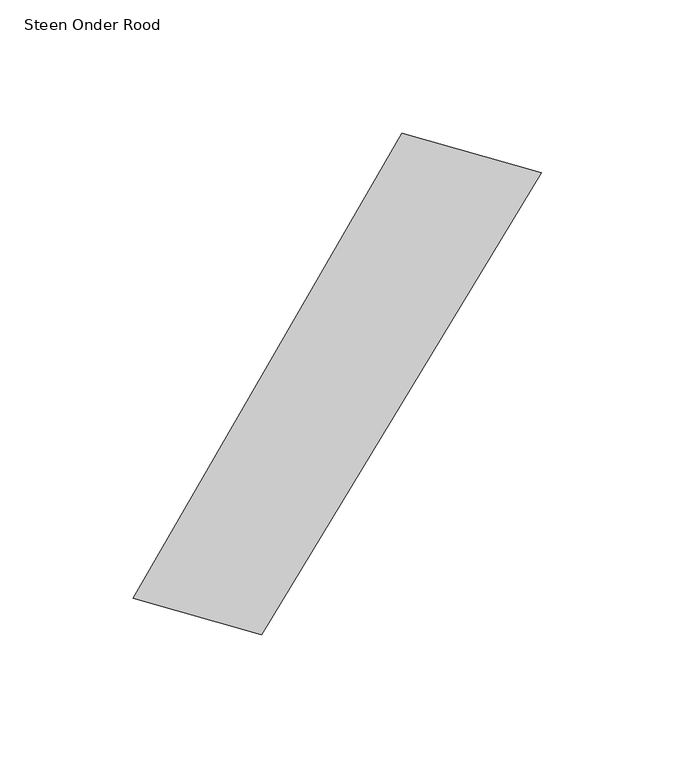
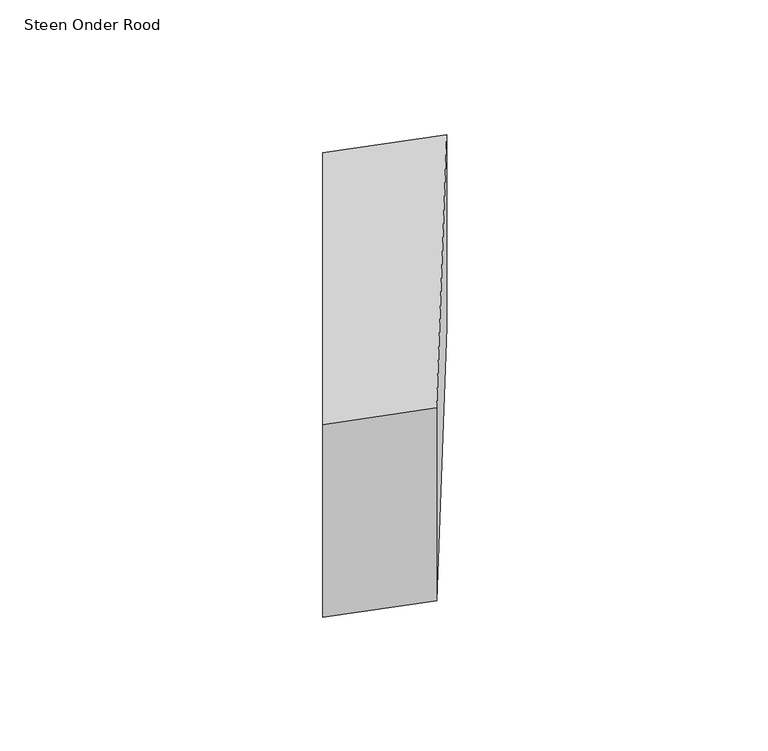
"""IFC4 building model written with IfcOpenShell, lengths in millimetres: proxy geometry, 00_GMA_steen_versie_4 : Steen Onder Rood."""

import ifcopenshell
import ifcopenshell.guid

model = None  # the IFC model being written
_history = None  # IfcOwnerHistory: only IFC2X3 demands one
_inside = {}  # id of a spatial element -> (the spatial element, [elements in it])
_under = {}  # id of a project, library or spatial element -> (it, [spatial elements below it])
_declared = {}  # id of a project -> (the project, [libraries it declares])
_typed = {}  # id of a type object -> (the type object, [elements of that type])
_made_of = {}  # id of a material, layer set ... -> (it, [elements and type objects made of it])


def new_model(schema):
    """Start an empty IFC model of exactly this schema.

    Asked for "IFC4X3", IfcOpenShell would pick the latest addendum, in which some entities
    have other attributes; the version numbers below select the first issue.
    IFC2X3 requires an IfcOwnerHistory on every rooted entity: one is made here for all.
    """
    global model, _history
    if schema == "IFC4X3":
        model = ifcopenshell.file(schema_version=(4, 3, 0, 0))
    else:
        model = ifcopenshell.file(schema=schema)
    _inside.clear()
    _under.clear()
    _declared.clear()
    _typed.clear()
    _made_of.clear()
    _history = None
    if model.schema == "IFC2X3":
        org = make("IfcOrganization", Name="unknown")
        user = make(
            "IfcPersonAndOrganization",
            ThePerson=make("IfcPerson", FamilyName="unknown"),
            TheOrganization=org,
        )
        app = make(
            "IfcApplication",
            ApplicationDeveloper=org,
            Version="unknown",
            ApplicationFullName="unknown",
            ApplicationIdentifier="unknown",
        )
        _history = make(
            "IfcOwnerHistory",
            OwningUser=user,
            OwningApplication=app,
            ChangeAction="ADDED",
            CreationDate=0,
        )
    return model


def make(cls, **values):
    """One entity of the class cls with the attributes given. An attribute that is None is left unset."""
    return model.create_entity(
        cls, **{name: value for name, value in values.items() if value is not None}
    )


def rooted(cls, **values):
    """An entity with a GlobalId (a new one), such as an element, a storey or a relation."""
    return make(cls, GlobalId=ifcopenshell.guid.new(), OwnerHistory=_history, **values)


def si_unit(unit_type, name, prefix=None):
    """IfcSIUnit, for example si_unit("LENGTHUNIT", "METRE", prefix="MILLI")."""
    return make("IfcSIUnit", UnitType=unit_type, Prefix=prefix, Name=name)


def assignment(units):
    """IfcUnitAssignment: the units of a project."""
    return None if units is None else make("IfcUnitAssignment", Units=units)


def point(xyz):
    """IfcCartesianPoint."""
    return None if xyz is None else make("IfcCartesianPoint", Coordinates=xyz)


def direction(xyz):
    """IfcDirection."""
    return None if xyz is None else make("IfcDirection", DirectionRatios=xyz)


def frame(location, z_axis=None, x_axis=None):
    """IfcAxis2Placement3D, a coordinate frame: its origin and axes. An axis left out is left unset."""
    return make(
        "IfcAxis2Placement3D",
        Location=point(location),
        Axis=direction(z_axis),
        RefDirection=direction(x_axis),
    )


def origin():
    """The frame at (0, 0, 0) with its axes left unset."""
    return frame((0.0, 0.0, 0.0))


def origin_with_axes():
    """The frame at (0, 0, 0) with the z axis (0, 0, 1) and the x axis (1, 0, 0) written out."""
    return frame((0.0, 0.0, 0.0), z_axis=(0.0, 0.0, 1.0), x_axis=(1.0, 0.0, 0.0))


def place(relative_to, where):
    """IfcLocalPlacement: puts the frame where relative to a parent placement (None: the world)."""
    return make(
        "IfcLocalPlacement", PlacementRelTo=relative_to, RelativePlacement=where
    )


def context(
    kind, dimensions, precision=None, world=None, true_north=None, identifier=None
):
    """IfcGeometricRepresentationContext, for example the 3D "Model" context."""
    return make(
        "IfcGeometricRepresentationContext",
        ContextIdentifier=identifier,
        ContextType=kind,
        CoordinateSpaceDimension=dimensions,
        Precision=precision,
        WorldCoordinateSystem=world,
        TrueNorth=true_north,
    )


def project(units=None, contexts=None):
    """IfcProject with its units and contexts."""
    return rooted(
        "IfcProject",
        Name="project",
        RepresentationContexts=contexts,
        UnitsInContext=assignment(units),
    )


def spatial(cls, under=None, at=None, **own):
    """A site, building, storey or space (cls), placed at a placement, below another one or the project."""
    s = rooted(cls, ObjectPlacement=at, **own)
    if under is not None:
        _under.setdefault(under.id(), (under, []))[1].append(s)
    return s


def polyline(points):
    """IfcPolyline through the points."""
    return make("IfcPolyline", Points=[point(p) for p in points])


def outline(outer, holes=None, kind="AREA"):
    """IfcArbitraryClosedProfileDef: a profile drawn as a closed curve; with holes, ...WithVoids."""
    if holes is None:
        return make("IfcArbitraryClosedProfileDef", ProfileType=kind, OuterCurve=outer)
    return make(
        "IfcArbitraryProfileDefWithVoids",
        ProfileType=kind,
        OuterCurve=outer,
        InnerCurves=holes,
    )


def extrude(swept, where, along, depth):
    """IfcExtrudedAreaSolid: the profile swept, set in the frame where, extruded along a direction by depth."""
    return make(
        "IfcExtrudedAreaSolid",
        SweptArea=swept,
        Position=where,
        ExtrudedDirection=direction(along),
        Depth=depth,
    )


def shape(context_of_items, identifier, shape_type, items):
    """IfcShapeRepresentation: the items that make up one representation, for example the "Body"."""
    return make(
        "IfcShapeRepresentation",
        ContextOfItems=context_of_items,
        RepresentationIdentifier=identifier,
        RepresentationType=shape_type,
        Items=items,
    )


def source(mapping_origin, context_of_items, identifier, shape_type, items):
    """IfcRepresentationMap: a shape defined once, which mapped items show again and again."""
    return make(
        "IfcRepresentationMap",
        MappingOrigin=mapping_origin,
        MappedRepresentation=shape(context_of_items, identifier, shape_type, items),
    )


def transform(
    local_origin,
    x_axis=None,
    y_axis=None,
    z_axis=None,
    scale=None,
    scale2=None,
    scale3=None,
    uniform=True,
):
    """IfcCartesianTransformationOperator3D, or its non-uniform kind. x_axis, y_axis, z_axis: its Axis1, 2, 3."""
    if uniform:
        return make(
            "IfcCartesianTransformationOperator3D",
            Axis1=direction(x_axis),
            Axis2=direction(y_axis),
            LocalOrigin=point(local_origin),
            Scale=scale,
            Axis3=direction(z_axis),
        )
    return make(
        "IfcCartesianTransformationOperator3DnonUniform",
        Axis1=direction(x_axis),
        Axis2=direction(y_axis),
        LocalOrigin=point(local_origin),
        Scale=scale,
        Axis3=direction(z_axis),
        Scale2=scale2,
        Scale3=scale3,
    )


def mapped(mapping_source, mapping_target):
    """IfcMappedItem: shows the shape of a source again, moved by a transform."""
    return make(
        "IfcMappedItem", MappingSource=mapping_source, MappingTarget=mapping_target
    )


def made_of(thing, what):
    """Note that an element or type object is made of a material, layer set ...; save() writes the relation."""
    if what is not None:
        _made_of.setdefault(what.id(), (what, []))[1].append(thing)
    return thing


def element(
    cls,
    number,
    at=None,
    inside=None,
    cuts=None,
    type_object=None,
    material=None,
    context=None,
    identifier="Body",
    shape_type=None,
    held_by="IfcProductDefinitionShape",
    body=None,
    shapes=None,
    **own,
):
    """One element of the class cls, such as IfcWall. Its Tag is "e" and its number.

    at: its placement. inside: the storey or other place that contains it. cuts: it is an
    opening in that element (IfcRelVoidsElement). A single representation is given by context,
    identifier, shape_type and body (its items); several are given by shapes. held_by: the class
    of the entity that holds the representations. save() writes the other relations.
    """
    e = rooted(cls, Tag="e%d" % number, ObjectPlacement=at, **own)
    if body is not None:
        shapes = [shape(context, identifier, shape_type, body)]
    if shapes is not None:
        e.Representation = make(held_by, Representations=shapes)
    if inside is not None:
        _inside.setdefault(inside.id(), (inside, []))[1].append(e)
    if cuts is not None:
        rooted(
            "IfcRelVoidsElement", RelatingBuildingElement=cuts, RelatedOpeningElement=e
        )
    if type_object is not None:
        _typed.setdefault(type_object.id(), (type_object, []))[1].append(e)
    return made_of(e, material)


def aggregate(whole, parts):
    """IfcRelAggregates: a whole, such as a stair, and the parts it consists of."""
    return rooted("IfcRelAggregates", RelatingObject=whole, RelatedObjects=parts)


def save(model, path):
    """Write the relations noted so far, then the file.

    IfcRelAggregates (storeys below a building ...), IfcRelContainedInSpatialStructure (elements
    in a storey), IfcRelDefinesByType, IfcRelAssociatesMaterial and IfcRelDeclares: one each for
    every whole, place, type object, material and project.
    """
    for whole, parts in _under.values():
        aggregate(whole, parts)
    for where, things in _inside.values():
        rooted(
            "IfcRelContainedInSpatialStructure",
            RelatedElements=things,
            RelatingStructure=where,
        )
    for kind, things in _typed.values():
        rooted("IfcRelDefinesByType", RelatedObjects=things, RelatingType=kind)
    for what, things in _made_of.values():
        rooted("IfcRelAssociatesMaterial", RelatedObjects=things, RelatingMaterial=what)
    for by, libraries in _declared.values():
        rooted("IfcRelDeclares", RelatingContext=by, RelatedDefinitions=libraries)
    model.write(path)


def steen_onder_rood_00cee3c2(model_context):
    return source(origin(), model_context, "Body", "SweptSolid", [
        extrude(outline(polyline([(151.9565091, 154.4198212), (46.9301943, -18.7978323), (-1.2031551, -5.2634066), (99.6350154, 169.1084483), (151.9565091, 154.4198212)])), origin_with_axes(), (0.0, 0.0, 1.0), 100.0),
    ])


if __name__ == "__main__":
    model = new_model("IFC4")
    model_context = context("Model", 3, world=origin())
    ifc_project = project(units=[si_unit("LENGTHUNIT", "METRE", prefix="MILLI")], contexts=[model_context])
    site = spatial("IfcSite", under=ifc_project)
    building = spatial("IfcBuilding", under=site)
    placement = place(None, origin())
    steen_onder_rood_shape = steen_onder_rood_00cee3c2(model_context)
    element("IfcBuildingElementProxy", 1, Name="00_GMA_steen_versie_4 : Steen Onder Rood", ObjectType="00_GMA_steen_versie_4 : Steen Onder Rood", at=placement, inside=building, context=model_context, shape_type="MappedRepresentation", body=[
        mapped(steen_onder_rood_shape, transform((0.0, 0.0, 0.0), x_axis=(1.0, 0.0, 0.0), y_axis=(0.0, 1.0, 0.0), z_axis=(0.0, 0.0, 1.0))),
    ])
    save(model, "model.ifc")

# Revit data of these elements
# Type "00_GMA_steen_versie_4 : Steen Onder Rood"
#   StootVoegHalfBoven [instance default] = 5 mm
#   StootVoegHalf [instance default] = 5 mm
#   StootVoegBreedteOnder = 10 mm
#   StootVoegBreedteBoven = 10 mm
#   Steendikte = 100 mm
#   LintVoegOnderHalf = 0 mm
#   LintVoegOnder = 0 mm
#   LintVoegBovenHalf = 5 mm
#   LintVoegBoven = 10 mm
#   materiaal = 21_steen_rood
#   MateriaalVoeg = none
#   Default Elevation = 0
# Element 1 (IfcBuildingElementProxy, "00_GMA_steen_versie_4 : Steen Onder Rood")
#   Materials on its faces: "21_steen_rood"
# Materials
#   "21_steen_rood": class "Unassigned", colour RGB 213 111 43, transparency 0, Cost = 0
